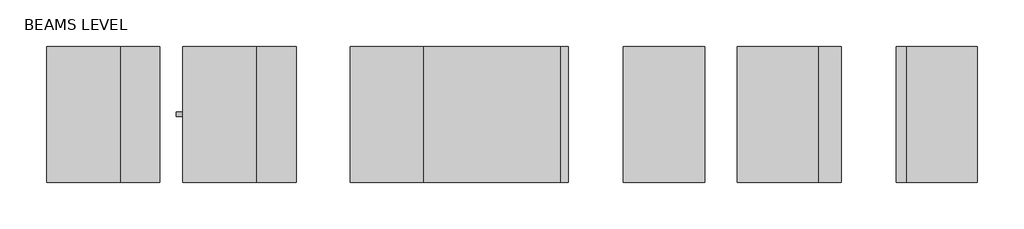
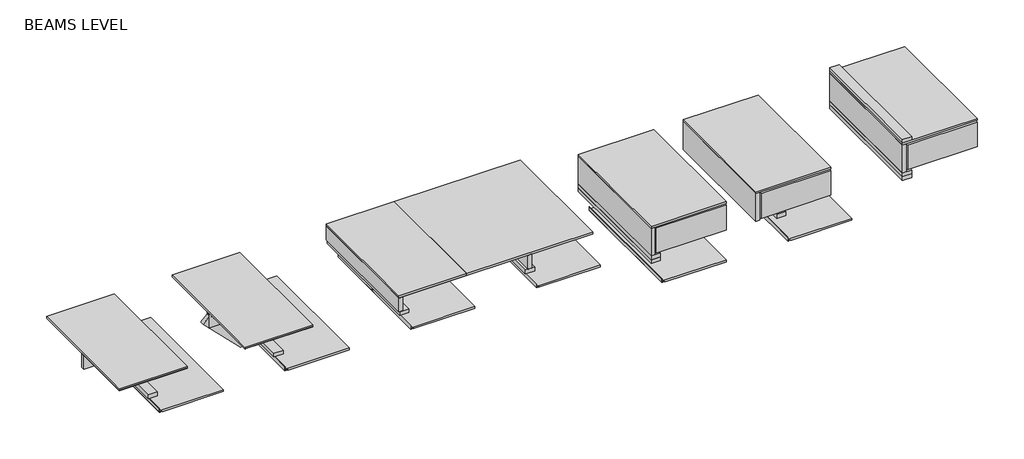
# One storey: 59 proxies.
"""IFC4 building model written with IfcOpenShell, lengths in millimetres."""

import ifcopenshell
import ifcopenshell.guid

model = None  # the IFC model being written
_history = None  # IfcOwnerHistory: only IFC2X3 demands one
_inside = {}  # id of a spatial element -> (the spatial element, [elements in it])
_under = {}  # id of a project, library or spatial element -> (it, [spatial elements below it])
_declared = {}  # id of a project -> (the project, [libraries it declares])
_typed = {}  # id of a type object -> (the type object, [elements of that type])
_made_of = {}  # id of a material, layer set ... -> (it, [elements and type objects made of it])


def new_model(schema):
    """Start an empty IFC model of exactly this schema.

    Asked for "IFC4X3", IfcOpenShell would pick the latest addendum, in which some entities
    have other attributes; the version numbers below select the first issue.
    IFC2X3 requires an IfcOwnerHistory on every rooted entity: one is made here for all.
    """
    global model, _history
    if schema == "IFC4X3":
        model = ifcopenshell.file(schema_version=(4, 3, 0, 0))
    else:
        model = ifcopenshell.file(schema=schema)
    _inside.clear()
    _under.clear()
    _declared.clear()
    _typed.clear()
    _made_of.clear()
    _history = None
    if model.schema == "IFC2X3":
        org = make("IfcOrganization", Name="unknown")
        user = make(
            "IfcPersonAndOrganization",
            ThePerson=make("IfcPerson", FamilyName="unknown"),
            TheOrganization=org,
        )
        app = make(
            "IfcApplication",
            ApplicationDeveloper=org,
            Version="unknown",
            ApplicationFullName="unknown",
            ApplicationIdentifier="unknown",
        )
        _history = make(
            "IfcOwnerHistory",
            OwningUser=user,
            OwningApplication=app,
            ChangeAction="ADDED",
            CreationDate=0,
        )
    return model


def make(cls, **values):
    """One entity of the class cls with the attributes given. An attribute that is None is left unset."""
    return model.create_entity(
        cls, **{name: value for name, value in values.items() if value is not None}
    )


def rooted(cls, **values):
    """An entity with a GlobalId (a new one), such as an element, a storey or a relation."""
    return make(cls, GlobalId=ifcopenshell.guid.new(), OwnerHistory=_history, **values)


def si_unit(unit_type, name, prefix=None):
    """IfcSIUnit, for example si_unit("LENGTHUNIT", "METRE", prefix="MILLI")."""
    return make("IfcSIUnit", UnitType=unit_type, Prefix=prefix, Name=name)


def assignment(units):
    """IfcUnitAssignment: the units of a project."""
    return None if units is None else make("IfcUnitAssignment", Units=units)


def point(xyz):
    """IfcCartesianPoint."""
    return None if xyz is None else make("IfcCartesianPoint", Coordinates=xyz)


def direction(xyz):
    """IfcDirection."""
    return None if xyz is None else make("IfcDirection", DirectionRatios=xyz)


def frame(location, z_axis=None, x_axis=None):
    """IfcAxis2Placement3D, a coordinate frame: its origin and axes. An axis left out is left unset."""
    return make(
        "IfcAxis2Placement3D",
        Location=point(location),
        Axis=direction(z_axis),
        RefDirection=direction(x_axis),
    )


def origin():
    """The frame at (0, 0, 0) with its axes left unset."""
    return frame((0.0, 0.0, 0.0))


def place(relative_to, where):
    """IfcLocalPlacement: puts the frame where relative to a parent placement (None: the world)."""
    return make(
        "IfcLocalPlacement", PlacementRelTo=relative_to, RelativePlacement=where
    )


def context(
    kind, dimensions, precision=None, world=None, true_north=None, identifier=None
):
    """IfcGeometricRepresentationContext, for example the 3D "Model" context."""
    return make(
        "IfcGeometricRepresentationContext",
        ContextIdentifier=identifier,
        ContextType=kind,
        CoordinateSpaceDimension=dimensions,
        Precision=precision,
        WorldCoordinateSystem=world,
        TrueNorth=true_north,
    )


def project(units=None, contexts=None):
    """IfcProject with its units and contexts."""
    return rooted(
        "IfcProject",
        Name="project",
        RepresentationContexts=contexts,
        UnitsInContext=assignment(units),
    )


def spatial(cls, under=None, at=None, **own):
    """A site, building, storey or space (cls), placed at a placement, below another one or the project."""
    s = rooted(cls, ObjectPlacement=at, **own)
    if under is not None:
        _under.setdefault(under.id(), (under, []))[1].append(s)
    return s


def polyline(points):
    """IfcPolyline through the points."""
    return make("IfcPolyline", Points=[point(p) for p in points])


def outline(outer, holes=None, kind="AREA"):
    """IfcArbitraryClosedProfileDef: a profile drawn as a closed curve; with holes, ...WithVoids."""
    if holes is None:
        return make("IfcArbitraryClosedProfileDef", ProfileType=kind, OuterCurve=outer)
    return make(
        "IfcArbitraryProfileDefWithVoids",
        ProfileType=kind,
        OuterCurve=outer,
        InnerCurves=holes,
    )


def extrude(swept, where, along, depth):
    """IfcExtrudedAreaSolid: the profile swept, set in the frame where, extruded along a direction by depth."""
    return make(
        "IfcExtrudedAreaSolid",
        SweptArea=swept,
        Position=where,
        ExtrudedDirection=direction(along),
        Depth=depth,
    )


def shape(context_of_items, identifier, shape_type, items):
    """IfcShapeRepresentation: the items that make up one representation, for example the "Body"."""
    return make(
        "IfcShapeRepresentation",
        ContextOfItems=context_of_items,
        RepresentationIdentifier=identifier,
        RepresentationType=shape_type,
        Items=items,
    )


def source(mapping_origin, context_of_items, identifier, shape_type, items):
    """IfcRepresentationMap: a shape defined once, which mapped items show again and again."""
    return make(
        "IfcRepresentationMap",
        MappingOrigin=mapping_origin,
        MappedRepresentation=shape(context_of_items, identifier, shape_type, items),
    )


def transform(
    local_origin,
    x_axis=None,
    y_axis=None,
    z_axis=None,
    scale=None,
    scale2=None,
    scale3=None,
    uniform=True,
):
    """IfcCartesianTransformationOperator3D, or its non-uniform kind. x_axis, y_axis, z_axis: its Axis1, 2, 3."""
    if uniform:
        return make(
            "IfcCartesianTransformationOperator3D",
            Axis1=direction(x_axis),
            Axis2=direction(y_axis),
            LocalOrigin=point(local_origin),
            Scale=scale,
            Axis3=direction(z_axis),
        )
    return make(
        "IfcCartesianTransformationOperator3DnonUniform",
        Axis1=direction(x_axis),
        Axis2=direction(y_axis),
        LocalOrigin=point(local_origin),
        Scale=scale,
        Axis3=direction(z_axis),
        Scale2=scale2,
        Scale3=scale3,
    )


def mapped(mapping_source, mapping_target):
    """IfcMappedItem: shows the shape of a source again, moved by a transform."""
    return make(
        "IfcMappedItem", MappingSource=mapping_source, MappingTarget=mapping_target
    )


def made_of(thing, what):
    """Note that an element or type object is made of a material, layer set ...; save() writes the relation."""
    if what is not None:
        _made_of.setdefault(what.id(), (what, []))[1].append(thing)
    return thing


def element(
    cls,
    number,
    at=None,
    inside=None,
    cuts=None,
    type_object=None,
    material=None,
    context=None,
    identifier="Body",
    shape_type=None,
    held_by="IfcProductDefinitionShape",
    body=None,
    shapes=None,
    **own,
):
    """One element of the class cls, such as IfcWall. Its Tag is "e" and its number.

    at: its placement. inside: the storey or other place that contains it. cuts: it is an
    opening in that element (IfcRelVoidsElement). A single representation is given by context,
    identifier, shape_type and body (its items); several are given by shapes. held_by: the class
    of the entity that holds the representations. save() writes the other relations.
    """
    e = rooted(cls, Tag="e%d" % number, ObjectPlacement=at, **own)
    if body is not None:
        shapes = [shape(context, identifier, shape_type, body)]
    if shapes is not None:
        e.Representation = make(held_by, Representations=shapes)
    if inside is not None:
        _inside.setdefault(inside.id(), (inside, []))[1].append(e)
    if cuts is not None:
        rooted(
            "IfcRelVoidsElement", RelatingBuildingElement=cuts, RelatedOpeningElement=e
        )
    if type_object is not None:
        _typed.setdefault(type_object.id(), (type_object, []))[1].append(e)
    return made_of(e, material)


def aggregate(whole, parts):
    """IfcRelAggregates: a whole, such as a stair, and the parts it consists of."""
    return rooted("IfcRelAggregates", RelatingObject=whole, RelatedObjects=parts)


def save(model, path):
    """Write the relations noted so far, then the file.

    IfcRelAggregates (storeys below a building ...), IfcRelContainedInSpatialStructure (elements
    in a storey), IfcRelDefinesByType, IfcRelAssociatesMaterial and IfcRelDeclares: one each for
    every whole, place, type object, material and project.
    """
    for whole, parts in _under.values():
        aggregate(whole, parts)
    for where, things in _inside.values():
        rooted(
            "IfcRelContainedInSpatialStructure",
            RelatedElements=things,
            RelatingStructure=where,
        )
    for kind, things in _typed.values():
        rooted("IfcRelDefinesByType", RelatedObjects=things, RelatingType=kind)
    for what, things in _made_of.values():
        rooted("IfcRelAssociatesMaterial", RelatedObjects=things, RelatingMaterial=what)
    for by, libraries in _declared.values():
        rooted("IfcRelDeclares", RelatingContext=by, RelatedDefinitions=libraries)
    model.write(path)


def generic_models_10_generic_models_1_ea081297(model_context):
    return source(origin(), model_context, "Body", "SweptSolid", [
        extrude(outline(polyline([(49758.6, 0.0), (49720.5, 0.0), (49720.5, 1219.2), (49758.6, 1219.2), (49758.6, 0.0)])), frame((0.0, 0.0, 5507.83125), z_axis=(0.0, 0.0, 1.0), x_axis=(1.0, 0.0, 0.0)), (0.0, 0.0, 1.0), 139.7),
    ])


def generic_models_109_generic_models_1_8619d77b(model_context):
    return source(origin(), model_context, "Body", "SweptSolid", [
        extrude(outline(polyline([(51003.2, 0.0), (50914.3, 0.0), (50914.3, 1219.2), (51003.2, 1219.2), (51003.2, 0.0)])), frame((0.0, 0.0, 5184.378125), z_axis=(0.0, 0.0, 1.0), x_axis=(1.0, 0.0, 0.0)), (0.0, 0.0, 1.0), 38.1),
    ])


def generic_models_110_generic_models_1_6bdce9b6(model_context):
    return source(origin(), model_context, "Body", "SweptSolid", [
        extrude(outline(polyline([(51642.1451407, 1219.2), (51642.1451407, 0.0), (50914.3, 0.0), (50914.3, 1219.2), (51642.1451407, 1219.2)])), frame((0.0, 0.0, 5508.228125), z_axis=(0.0, 0.0, 1.0), x_axis=(1.0, 0.0, 0.0)), (0.0, 0.0, 1.0), 19.05),
    ])


def generic_models_112_generic_models_65_d168d7b0(model_context):
    return source(origin(), model_context, "Body", "SweptSolid", [
        extrude(outline(polyline([(50952.4, 592.1375), (50952.4, 630.2375), (51642.1451407, 630.2375), (51642.1451407, 592.1375), (50952.4, 592.1375)])), frame((0.0, 0.0, 5222.478125), z_axis=(0.0, 0.0, 1.0), x_axis=(1.0, 0.0, 0.0)), (0.0, 0.0, 1.0), 285.75),
    ])


def generic_models_113_generic_models_1_101608ab(model_context):
    return source(origin(), model_context, "Body", "SweptSolid", [
        extrude(outline(polyline([(52171.6, 0.0), (52133.5, 0.0), (52133.5, 1219.2), (52171.6, 1219.2), (52171.6, 0.0)])), frame((0.0, 0.0, 5222.478125), z_axis=(0.0, 0.0, 1.0), x_axis=(1.0, 0.0, 0.0)), (0.0, 0.0, 1.0), 285.75),
    ])


def generic_models_114_generic_models_1_a6fb1c2c(model_context):
    return source(origin(), model_context, "Body", "SweptSolid", [
        extrude(outline(polyline([(51642.1451407, 1219.2), (51642.1451407, 0.0), (50965.9242022, 0.0), (50965.9242022, 1219.2), (51642.1451407, 1219.2)])), frame((0.0, 0.0, 5237.6235034), z_axis=(0.0, 0.0, 1.0), x_axis=(1.0, 0.0, 0.0)), (0.0, 0.0, 1.0), 254.0),
    ])


def generic_models_12_generic_models_46_b8a9a4e8(model_context):
    return source(origin(), model_context, "Body", "SweptSolid", [
        extrude(outline(polyline([(49757.8505137, 0.0), (49721.1284797, 0.0), (49721.1284797, 1219.2), (49757.8505137, 1219.2), (49757.8505137, 0.0)])), frame((0.0, 0.0, 5505.7509163), z_axis=(0.0, 0.0, 1.0), x_axis=(1.0, 0.0, 0.0)), (0.0, 0.0, 1.0), 1.5875),
    ])


def generic_models_13_generic_models_65_9e643fb9(model_context):
    return source(origin(), model_context, "Body", "SweptSolid", [
        extrude(outline(polyline([(49128.3625, 592.1375), (49128.3625, 630.2375), (50347.5625, 630.2375), (50347.5625, 592.1375), (49128.3625, 592.1375)])), frame((0.0, 0.0, 5507.83125), z_axis=(0.0, 0.0, 1.0), x_axis=(1.0, 0.0, 0.0)), (0.0, 0.0, 1.0), 139.7),
    ])


def generic_models_14_generic_models_1_e8c90d4c(model_context):
    return source(origin(), model_context, "Body", "SweptSolid", [
        extrude(outline(polyline([(2277.1204978, 49799.875), (2239.0204978, 49799.875), (2239.0204978, 49825.275), (2240.6079978, 49825.275), (2240.6079978, 49801.4625), (2277.1204978, 49801.4625), (2277.1204978, 49799.875)])), frame((0.0, 0.0, 0.0), z_axis=(0.0, 1.0, 0.0), x_axis=(0.0, 0.0, 1.0)), (0.0, 0.0, 1.0), 1219.2),
    ])


def generic_models_22_generic_models_1_e5767157(model_context):
    return source(origin(), model_context, "Body", "SweptSolid", [
        extrude(outline(polyline([(2409.6091, 49800.66875), (2409.6091, 49799.875), (2407.0592364, 49799.875), (2405.4618473, 49749.075), (2404.6631527, 49749.075), (2403.0657636, 49799.875), (2400.5159, 49799.875), (2400.5159, 49800.66875), (2409.6091, 49800.66875)])), frame((0.0, 565.15, 0.0), z_axis=(0.0, 1.0, 0.0), x_axis=(0.0, 0.0, 1.0)), (0.0, 0.0, 1.0), 12.7),
    ])


def generic_models_226_generic_models_1_7dc37832(model_context):
    return source(origin(), model_context, "Body", "SweptSolid", [
        extrude(outline(polyline([(5263.35625, 49733.4159), (5263.35625, 49742.5091), (5264.15, 49742.5091), (5264.15, 49739.9592364), (5314.95, 49738.3618473), (5314.95, 49737.5631527), (5264.15, 49735.9657636), (5264.15, 49733.4159), (5263.35625, 49733.4159)])), frame((0.0, 565.15, 0.0), z_axis=(0.0, 1.0, 0.0), x_axis=(0.0, 0.0, 1.0)), (0.0, 0.0, 1.0), 12.7),
    ])


def generic_models_202_generic_models_1_0ad20a8b(model_context):
    return source(origin(), model_context, "Body", "SweptSolid", [
        extrude(outline(polyline([(2253.330428, 49813.3451407), (2242.217928, 49813.3451407), (2242.217928, 49826.0451407), (2234.280428, 49828.9341545), (2234.280428, 50422.9451407), (2253.330428, 50422.9451407), (2253.330428, 49813.3451407)])), frame((0.0, 0.0, 0.0), z_axis=(0.0, 1.0, 0.0), x_axis=(0.0, 0.0, 1.0)), (0.0, 0.0, 1.0), 1219.2),
    ])


def generic_models_233_generic_models_1_ae5bae41(model_context):
    return source(origin(), model_context, "Body", "SweptSolid", [
        extrude(outline(polyline([(48564.8, 0.0), (48475.9, 0.0), (48475.9, 1219.2), (48564.8, 1219.2), (48564.8, 0.0)])), frame((0.0, 0.0, 5467.35), z_axis=(0.0, 0.0, 1.0), x_axis=(1.0, 0.0, 0.0)), (0.0, 0.0, 1.0), 38.1),
    ])


def generic_models_236_generic_models_1_f8917e71(model_context):
    return source(origin(), model_context, "Body", "SweptSolid", [
        extrude(outline(polyline([(48507.65, 0.0), (48469.55, 0.0), (48469.55, 1219.2), (48507.65, 1219.2), (48507.65, 0.0)])), frame((0.0, 0.0, 5507.83125), z_axis=(0.0, 0.0, 1.0), x_axis=(1.0, 0.0, 0.0)), (0.0, 0.0, 1.0), 139.7),
    ])


def generic_models_237_generic_models_65_1df05f16(model_context):
    return source(origin(), model_context, "Body", "SweptSolid", [
        extrude(outline(polyline([(48469.55, 592.1375), (48469.55, 630.2375), (49128.3625, 630.2375), (49128.3625, 592.1375), (48469.55, 592.1375)])), frame((0.0, 0.0, 5507.83125), z_axis=(0.0, 0.0, 1.0), x_axis=(1.0, 0.0, 0.0)), (0.0, 0.0, 1.0), 139.7),
    ])


def generic_models_239_generic_models_46_95e6735a(model_context):
    return source(origin(), model_context, "Body", "SweptSolid", [
        extrude(outline(polyline([(50347.5625, 0.0), (49691.4320511, 0.0), (49691.4320511, 1219.2), (50347.5625, 1219.2), (50347.5625, 0.0)])), frame((0.0, 0.0, 5505.7509163), z_axis=(0.0, 0.0, 1.0), x_axis=(1.0, 0.0, 0.0)), (0.0, 0.0, 1.0), 1.5875),
    ])


def generic_models_240_generic_models_1_611786cf(model_context):
    return source(origin(), model_context, "Body", "SweptSolid", [
        extrude(outline(polyline([(49128.3625, 1219.2), (49128.3625, 0.0), (48469.55, 0.0), (48469.55, 1219.2), (49128.3625, 1219.2)])), frame((0.0, 0.0, 5649.9125), z_axis=(0.0, 0.0, 1.0), x_axis=(1.0, 0.0, 0.0)), (0.0, 0.0, 1.0), 19.05),
    ])


def generic_models_267_generic_models_65_11354230(model_context):
    return source(origin(), model_context, "Body", "SweptSolid", [
        extrude(outline(polyline([(0.0, -38.1), (0.0, 0.0), (514.35, 0.0), (514.35, -38.1), (0.0, -38.1)])), frame((47276.4596037, 592.1375, 5202.484661), z_axis=(0.7071067811865633, 0.0, 0.7071067811865317), x_axis=(-0.7071067811865317, 0.0, 0.7071067811865633)), (0.0, 0.0, 1.0), 88.9),
    ])


def generic_models_29_generic_models_1_59087225(model_context):
    return source(origin(), model_context, "Body", "SweptSolid", [
        extrude(outline(polyline([(50347.5625, 1219.2), (50347.5625, 0.0), (49128.3625, 0.0), (49128.3625, 1219.2), (50347.5625, 1219.2)])), frame((0.0, 0.0, 5647.53125), z_axis=(0.0, 0.0, 1.0), x_axis=(1.0, 0.0, 0.0)), (0.0, 0.0, 1.0), 19.05),
    ])


def generic_models_37_generic_models_1_916dd7c6(model_context):
    return source(origin(), model_context, "Body", "SweptSolid", [
        extrude(outline(polyline([(2409.6091, 49675.25625), (2400.5159, 49675.25625), (2400.5159, 49676.05), (2403.0657636, 49676.05), (2404.6631527, 49726.85), (2405.4618473, 49726.85), (2407.0592364, 49676.05), (2409.6091, 49676.05), (2409.6091, 49675.25625)])), frame((0.0, 565.15, 0.0), z_axis=(0.0, 1.0, 0.0), x_axis=(0.0, 0.0, 1.0)), (0.0, 0.0, 1.0), 12.7),
    ])


def generic_models_103_generic_models_1_250a6a11(model_context):
    return source(origin(), model_context, "Body", "SweptSolid", [
        extrude(outline(polyline([(49784.0, 0.0), (49695.1, 0.0), (49695.1, 1219.2), (49784.0, 1219.2), (49784.0, 0.0)])), frame((0.0, 0.0, 5264.15), z_axis=(0.0, 0.0, 1.0), x_axis=(1.0, 0.0, 0.0)), (0.0, 0.0, 1.0), 38.1),
    ])


def generic_models_71_generic_models_1_508a995f(model_context):
    return source(origin(), model_context, "Body", "SweptSolid", [
        extrude(outline(polyline([(50952.4, 0.0), (50914.3, 0.0), (50914.3, 1219.2), (50952.4, 1219.2), (50952.4, 0.0)])), frame((0.0, 0.0, 5222.478125), z_axis=(0.0, 0.0, 1.0), x_axis=(1.0, 0.0, 0.0)), (0.0, 0.0, 1.0), 285.75),
    ])


def generic_models_87_generic_models_1_55a64953(model_context):
    return source(origin(), model_context, "Body", "SweptSolid", [
        extrude(outline(polyline([(51968.4, 0.0), (51930.3, 0.0), (51930.3, 1219.2), (51968.4, 1219.2), (51968.4, 0.0)])), frame((0.0, 0.0, 5222.478125), z_axis=(0.0, 0.0, 1.0), x_axis=(1.0, 0.0, 0.0)), (0.0, 0.0, 1.0), 285.75),
    ])


model = new_model("IFC4")

# Units and contexts
model_context = context("Model", 3, world=origin())
ifc_project = project(units=[si_unit("LENGTHUNIT", "METRE", prefix="MILLI")], contexts=[model_context])

# Site, building, storey
site = spatial("IfcSite", under=ifc_project)
building = spatial("IfcBuilding", under=site)
storey = spatial("IfcBuildingStorey", under=building, Name="BEAMS LEVEL", Elevation=4876.8)

# Proxies
placement = place(None, origin())
generic_models_10_generic_models_1_shape = generic_models_10_generic_models_1_ea081297(model_context)
element("IfcBuildingElementProxy", 1, Name="Generic Models 10 : Generic Models 1", ObjectType="Generic Models 10 : Generic Models 1", at=placement, inside=storey, context=model_context, shape_type="MappedRepresentation", body=[
    mapped(generic_models_10_generic_models_1_shape, transform((0.0, 0.0, 0.0), x_axis=(1.0, 0.0, 0.0), y_axis=(0.0, 1.0, 0.0), z_axis=(0.0, 0.0, 1.0))),
])
generic_models_109_generic_models_1_shape = generic_models_109_generic_models_1_8619d77b(model_context)
element("IfcBuildingElementProxy", 2, Name="Generic Models 109 : Generic Models 1", ObjectType="Generic Models 109 : Generic Models 1", at=placement, inside=storey, context=model_context, shape_type="MappedRepresentation", body=[
    mapped(generic_models_109_generic_models_1_shape, transform((2438.4, 0.0, 0.0), x_axis=(1.0, 0.0, 0.0), y_axis=(0.0, 1.0, 0.0), z_axis=(0.0, 0.0, 1.0))),
])
generic_models_110_generic_models_1_shape = generic_models_110_generic_models_1_6bdce9b6(model_context)
element("IfcBuildingElementProxy", 3, Name="Generic Models 110 : Generic Models 1", ObjectType="Generic Models 110 : Generic Models 1", at=placement, inside=storey, context=model_context, shape_type="MappedRepresentation", body=[
    mapped(generic_models_110_generic_models_1_shape, transform((2438.4, 0.0, 0.0), x_axis=(1.0, 0.0, 0.0), y_axis=(0.0, 1.0, 0.0), z_axis=(0.0, 0.0, 1.0))),
])
element("IfcBuildingElementProxy", 4, Name="Generic Models 111 : Generic Models 1", ObjectType="Generic Models 111 : Generic Models 1", at=placement, inside=storey, context=model_context, shape_type="MappedRepresentation", body=[
    mapped(generic_models_109_generic_models_1_shape, transform((2438.4, 0.0, -38.1), x_axis=(1.0, 0.0, 0.0), y_axis=(0.0, 1.0, 0.0), z_axis=(0.0, 0.0, 1.0))),
])
generic_models_112_generic_models_65_shape = generic_models_112_generic_models_65_d168d7b0(model_context)
element("IfcBuildingElementProxy", 5, Name="Generic Models 112 : Generic Models 65", ObjectType="Generic Models 112 : Generic Models 65", at=placement, inside=storey, context=model_context, shape_type="MappedRepresentation", body=[
    mapped(generic_models_112_generic_models_65_shape, transform((2438.4, 0.0, 0.0), x_axis=(1.0, 0.0, 0.0), y_axis=(0.0, 1.0, 0.0), z_axis=(0.0, 0.0, 1.0))),
])
generic_models_113_generic_models_1_shape = generic_models_113_generic_models_1_101608ab(model_context)
element("IfcBuildingElementProxy", 6, Name="Generic Models 113 : Generic Models 1", ObjectType="Generic Models 113 : Generic Models 1", at=placement, inside=storey, context=model_context, shape_type="MappedRepresentation", body=[
    mapped(generic_models_113_generic_models_1_shape, transform((1219.2, 0.0, 0.0), x_axis=(1.0, 0.0, 0.0), y_axis=(0.0, 1.0, 0.0), z_axis=(0.0, 0.0, 1.0))),
])
generic_models_114_generic_models_1_shape = generic_models_114_generic_models_1_a6fb1c2c(model_context)
element("IfcBuildingElementProxy", 7, Name="Generic Models 114 : Generic Models 1", ObjectType="Generic Models 114 : Generic Models 1", at=placement, inside=storey, context=model_context, shape_type="MappedRepresentation", body=[
    mapped(generic_models_114_generic_models_1_shape, transform((2438.4, 0.0, 0.0), x_axis=(1.0, 0.0, 0.0), y_axis=(0.0, 1.0, 0.0), z_axis=(0.0, 0.0, 1.0))),
])
element("IfcBuildingElementProxy", 8, Name="Generic Models 115 : Generic Models 1", ObjectType="Generic Models 115 : Generic Models 1", at=placement, inside=storey, context=model_context, shape_type="MappedRepresentation", body=[
    mapped(generic_models_109_generic_models_1_shape, transform((2438.4, 0.0, 342.9), x_axis=(1.0, 0.0, 0.0), y_axis=(0.0, 1.0, 0.0), z_axis=(0.0, 0.0, 1.0))),
])
generic_models_12_generic_models_46_shape = generic_models_12_generic_models_46_b8a9a4e8(model_context)
element("IfcBuildingElementProxy", 9, Name="Generic Models 12 : Generic Models 46", ObjectType="Generic Models 12 : Generic Models 46", at=placement, inside=storey, context=model_context, shape_type="MappedRepresentation", body=[
    mapped(generic_models_12_generic_models_46_shape, transform((0.0, 0.0, 0.0), x_axis=(1.0, 0.0, 0.0), y_axis=(0.0, 1.0, 0.0), z_axis=(0.0, 0.0, 1.0))),
])
generic_models_13_generic_models_65_shape = generic_models_13_generic_models_65_9e643fb9(model_context)
element("IfcBuildingElementProxy", 10, Name="Generic Models 13 : Generic Models 65", ObjectType="Generic Models 13 : Generic Models 65", at=placement, inside=storey, context=model_context, shape_type="MappedRepresentation", body=[
    mapped(generic_models_13_generic_models_65_shape, transform((0.0, 0.0, 0.0), x_axis=(1.0, 0.0, 0.0), y_axis=(0.0, 1.0, 0.0), z_axis=(0.0, 0.0, 1.0))),
])
generic_models_14_generic_models_1_shape = generic_models_14_generic_models_1_e8c90d4c(model_context)
element("IfcBuildingElementProxy", 11, Name="Generic Models 14 : Generic Models 1", ObjectType="Generic Models 14 : Generic Models 1", at=placement, inside=storey, context=model_context, shape_type="MappedRepresentation", body=[
    mapped(generic_models_14_generic_models_1_shape, transform((0.0, 0.0, 3050.778125), x_axis=(1.0, 0.0, 0.0), y_axis=(0.0, 1.0, 0.0), z_axis=(0.0, 0.0, 1.0))),
])
generic_models_22_generic_models_1_shape = generic_models_22_generic_models_1_e5767157(model_context)
element("IfcBuildingElementProxy", 12, Name="Generic Models 22 : Generic Models 1", ObjectType="Generic Models 22 : Generic Models 1", at=placement, inside=storey, context=model_context, shape_type="MappedRepresentation", body=[
    mapped(generic_models_22_generic_models_1_shape, transform((0.0, 0.0, 3081.3375), x_axis=(1.0, 0.0, 0.0), y_axis=(0.0, 1.0, 0.0), z_axis=(0.0, 0.0, 1.0))),
])
element("IfcBuildingElementProxy", 13, Name="Generic Models 224 : Generic Models 1", ObjectType="Generic Models 224 : Generic Models 1", at=placement, inside=storey, context=model_context, shape_type="MappedRepresentation", body=[
    mapped(generic_models_14_generic_models_1_shape, transform((-1217.6125, 0.0, 3050.778125), x_axis=(1.0, 0.0, 0.0), y_axis=(0.0, 1.0, 0.0), z_axis=(0.0, 0.0, 1.0))),
])
element("IfcBuildingElementProxy", 14, Name="Generic Models 225 : Generic Models 1", ObjectType="Generic Models 225 : Generic Models 1", at=placement, inside=storey, context=model_context, shape_type="MappedRepresentation", body=[
    mapped(generic_models_22_generic_models_1_shape, transform((-1219.2, 0.0, 2960.6875), x_axis=(1.0, 0.0, 0.0), y_axis=(0.0, 1.0, 0.0), z_axis=(0.0, 0.0, 1.0))),
])
generic_models_226_generic_models_1_shape = generic_models_226_generic_models_1_7dc37832(model_context)
element("IfcBuildingElementProxy", 15, Name="Generic Models 226 : Generic Models 1", ObjectType="Generic Models 226 : Generic Models 1", at=placement, inside=storey, context=model_context, shape_type="MappedRepresentation", body=[
    mapped(generic_models_226_generic_models_1_shape, transform((-1219.2, 0.0, 203.2), x_axis=(1.0, 0.0, 0.0), y_axis=(0.0, 1.0, 0.0), z_axis=(0.0, 0.0, 1.0))),
])
generic_models_202_generic_models_1_shape = generic_models_202_generic_models_1_0ad20a8b(model_context)
element("IfcBuildingElementProxy", 16, Name="Generic Models 231 : Generic Models 1", ObjectType="Generic Models 231 : Generic Models 1", at=placement, inside=storey, context=model_context, shape_type="MappedRepresentation", body=[
    mapped(generic_models_202_generic_models_1_shape, transform((-1217.6125, 0.0, 3050.778125), x_axis=(1.0, 0.0, 0.0), y_axis=(0.0, 1.0, 0.0), z_axis=(0.0, 0.0, 1.0))),
])
generic_models_233_generic_models_1_shape = generic_models_233_generic_models_1_ae5bae41(model_context)
element("IfcBuildingElementProxy", 17, Name="Generic Models 233 : Generic Models 1", ObjectType="Generic Models 233 : Generic Models 1", at=placement, inside=storey, context=model_context, shape_type="MappedRepresentation", body=[
    mapped(generic_models_233_generic_models_1_shape, transform((0.0, 0.0, 0.0), x_axis=(1.0, 0.0, 0.0), y_axis=(0.0, 1.0, 0.0), z_axis=(0.0, 0.0, 1.0))),
])
generic_models_236_generic_models_1_shape = generic_models_236_generic_models_1_f8917e71(model_context)
element("IfcBuildingElementProxy", 18, Name="Generic Models 236 : Generic Models 1", ObjectType="Generic Models 236 : Generic Models 1", at=placement, inside=storey, context=model_context, shape_type="MappedRepresentation", body=[
    mapped(generic_models_236_generic_models_1_shape, transform((0.0, 0.0, 0.0), x_axis=(1.0, 0.0, 0.0), y_axis=(0.0, 1.0, 0.0), z_axis=(0.0, 0.0, 1.0))),
])
generic_models_237_generic_models_65_shape = generic_models_237_generic_models_65_1df05f16(model_context)
element("IfcBuildingElementProxy", 19, Name="Generic Models 237 : Generic Models 65", ObjectType="Generic Models 237 : Generic Models 65", at=placement, inside=storey, context=model_context, shape_type="MappedRepresentation", body=[
    mapped(generic_models_237_generic_models_65_shape, transform((0.0, 0.0, 0.0), x_axis=(1.0, 0.0, 0.0), y_axis=(0.0, 1.0, 0.0), z_axis=(0.0, 0.0, 1.0))),
])
element("IfcBuildingElementProxy", 20, Name="Generic Models 238 : Generic Models 1", ObjectType="Generic Models 238 : Generic Models 1", at=placement, inside=storey, context=model_context, shape_type="MappedRepresentation", body=[
    mapped(generic_models_14_generic_models_1_shape, transform((-3656.0125, 0.0, 3050.778125), x_axis=(1.0, 0.0, 0.0), y_axis=(0.0, 1.0, 0.0), z_axis=(0.0, 0.0, 1.0))),
])
generic_models_239_generic_models_46_shape = generic_models_239_generic_models_46_95e6735a(model_context)
element("IfcBuildingElementProxy", 21, Name="Generic Models 239 : Generic Models 46", ObjectType="Generic Models 239 : Generic Models 46", at=placement, inside=storey, context=model_context, shape_type="MappedRepresentation", body=[
    mapped(generic_models_239_generic_models_46_shape, transform((-1219.2, 0.0, 142.08125), x_axis=(1.0, 0.0, 0.0), y_axis=(0.0, 1.0, 0.0), z_axis=(0.0, 0.0, 1.0))),
])
generic_models_240_generic_models_1_shape = generic_models_240_generic_models_1_611786cf(model_context)
element("IfcBuildingElementProxy", 22, Name="Generic Models 240 : Generic Models 1", ObjectType="Generic Models 240 : Generic Models 1", at=placement, inside=storey, context=model_context, shape_type="MappedRepresentation", body=[
    mapped(generic_models_240_generic_models_1_shape, transform((0.0, 0.0, 0.0), x_axis=(1.0, 0.0, 0.0), y_axis=(0.0, 1.0, 0.0), z_axis=(0.0, 0.0, 1.0))),
])
element("IfcBuildingElementProxy", 23, Name="Generic Models 242 : Generic Models 1", ObjectType="Generic Models 242 : Generic Models 1", at=placement, inside=storey, context=model_context, shape_type="MappedRepresentation", body=[
    mapped(generic_models_22_generic_models_1_shape, transform((-3657.6, 0.0, 2960.6875), x_axis=(1.0, 0.0, 0.0), y_axis=(0.0, 1.0, 0.0), z_axis=(0.0, 0.0, 1.0))),
])
element("IfcBuildingElementProxy", 24, Name="Generic Models 243 : Generic Models 1", ObjectType="Generic Models 243 : Generic Models 1", at=placement, inside=storey, context=model_context, shape_type="MappedRepresentation", body=[
    mapped(generic_models_226_generic_models_1_shape, transform((-3656.0125, 0.0, 203.2), x_axis=(1.0, 0.0, 0.0), y_axis=(0.0, 1.0, 0.0), z_axis=(0.0, 0.0, 1.0))),
])
element("IfcBuildingElementProxy", 25, Name="Generic Models 245 : Generic Models 1", ObjectType="Generic Models 245 : Generic Models 1", at=placement, inside=storey, context=model_context, shape_type="MappedRepresentation", body=[
    mapped(generic_models_202_generic_models_1_shape, transform((-3656.0125, 0.0, 3050.778125), x_axis=(1.0, 0.0, 0.0), y_axis=(0.0, 1.0, 0.0), z_axis=(0.0, 0.0, 1.0))),
])
element("IfcBuildingElementProxy", 26, Name="Generic Models 247 : Generic Models 1", ObjectType="Generic Models 247 : Generic Models 1", at=placement, inside=storey, context=model_context, shape_type="MappedRepresentation", body=[
    mapped(generic_models_233_generic_models_1_shape, transform((-2438.4, 0.0, 0.0), x_axis=(1.0, 0.0, 0.0), y_axis=(0.0, 1.0, 0.0), z_axis=(0.0, 0.0, 1.0))),
])
element("IfcBuildingElementProxy", 27, Name="Generic Models 25 : Generic Models 46", ObjectType="Generic Models 25 : Generic Models 46", at=placement, inside=storey, context=model_context, shape_type="MappedRepresentation", body=[
    mapped(generic_models_12_generic_models_46_shape, transform((0.0, 0.0, 142.08125), x_axis=(1.0, 0.0, 0.0), y_axis=(0.0, 1.0, 0.0), z_axis=(0.0, 0.0, 1.0))),
])
element("IfcBuildingElementProxy", 28, Name="Generic Models 250 : Generic Models 65", ObjectType="Generic Models 250 : Generic Models 65", at=placement, inside=storey, context=model_context, shape_type="MappedRepresentation", body=[
    mapped(generic_models_237_generic_models_65_shape, transform((-2714.8439208, 0.0, 0.0), x_axis=(1.0, 0.0, 0.0), y_axis=(0.0, 1.0, 0.0), z_axis=(0.0, 0.0, 1.0))),
])
element("IfcBuildingElementProxy", 29, Name="Generic Models 251 : Generic Models 46", ObjectType="Generic Models 251 : Generic Models 46", at=placement, inside=storey, context=model_context, shape_type="MappedRepresentation", body=[
    mapped(generic_models_239_generic_models_46_shape, transform((-3934.0439208, 0.0, 142.08125), x_axis=(1.0, 0.0, 0.0), y_axis=(0.0, 1.0, 0.0), z_axis=(0.0, 0.0, 1.0))),
])
element("IfcBuildingElementProxy", 30, Name="Generic Models 252 : Generic Models 1", ObjectType="Generic Models 252 : Generic Models 1", at=placement, inside=storey, context=model_context, shape_type="MappedRepresentation", body=[
    mapped(generic_models_240_generic_models_1_shape, transform((-2714.8439208, 0.0, 0.0), x_axis=(1.0, 0.0, 0.0), y_axis=(0.0, 1.0, 0.0), z_axis=(0.0, 0.0, 1.0))),
])
element("IfcBuildingElementProxy", 31, Name="Generic Models 255 : Generic Models 1", ObjectType="Generic Models 255 : Generic Models 1", at=placement, inside=storey, context=model_context, shape_type="MappedRepresentation", body=[
    mapped(generic_models_14_generic_models_1_shape, transform((-2436.8125, 0.0, 3050.778125), x_axis=(1.0, 0.0, 0.0), y_axis=(0.0, 1.0, 0.0), z_axis=(0.0, 0.0, 1.0))),
])
element("IfcBuildingElementProxy", 32, Name="Generic Models 256 : Generic Models 1", ObjectType="Generic Models 256 : Generic Models 1", at=placement, inside=storey, context=model_context, shape_type="MappedRepresentation", body=[
    mapped(generic_models_22_generic_models_1_shape, transform((-2438.4, 0.0, 2960.6875), x_axis=(1.0, 0.0, 0.0), y_axis=(0.0, 1.0, 0.0), z_axis=(0.0, 0.0, 1.0))),
])
element("IfcBuildingElementProxy", 33, Name="Generic Models 257 : Generic Models 1", ObjectType="Generic Models 257 : Generic Models 1", at=placement, inside=storey, context=model_context, shape_type="MappedRepresentation", body=[
    mapped(generic_models_226_generic_models_1_shape, transform((-2438.4, 0.0, 203.2), x_axis=(1.0, 0.0, 0.0), y_axis=(0.0, 1.0, 0.0), z_axis=(0.0, 0.0, 1.0))),
])
element("IfcBuildingElementProxy", 34, Name="Generic Models 259 : Generic Models 1", ObjectType="Generic Models 259 : Generic Models 1", at=placement, inside=storey, context=model_context, shape_type="MappedRepresentation", body=[
    mapped(generic_models_202_generic_models_1_shape, transform((-2436.8125, 0.0, 3050.778125), x_axis=(1.0, 0.0, 0.0), y_axis=(0.0, 1.0, 0.0), z_axis=(0.0, 0.0, 1.0))),
])
element("IfcBuildingElementProxy", 35, Name="Generic Models 261 : Generic Models 1", ObjectType="Generic Models 261 : Generic Models 1", at=placement, inside=storey, context=model_context, shape_type="MappedRepresentation", body=[
    mapped(generic_models_233_generic_models_1_shape, transform((-1219.2, 0.0, 0.0), x_axis=(1.0, 0.0, 0.0), y_axis=(0.0, 1.0, 0.0), z_axis=(0.0, 0.0, 1.0))),
])
element("IfcBuildingElementProxy", 36, Name="Generic Models 264 : Generic Models 65", ObjectType="Generic Models 264 : Generic Models 65", at=placement, inside=storey, context=model_context, shape_type="MappedRepresentation", body=[
    mapped(generic_models_237_generic_models_65_shape, transform((-1497.80625, 0.0, 0.0), x_axis=(1.0, 0.0, 0.0), y_axis=(0.0, 1.0, 0.0), z_axis=(0.0, 0.0, 1.0))),
])
element("IfcBuildingElementProxy", 37, Name="Generic Models 265 : Generic Models 46", ObjectType="Generic Models 265 : Generic Models 46", at=placement, inside=storey, context=model_context, shape_type="MappedRepresentation", body=[
    mapped(generic_models_239_generic_models_46_shape, transform((-2717.00625, 0.0, 142.08125), x_axis=(1.0, 0.0, 0.0), y_axis=(0.0, 1.0, 0.0), z_axis=(0.0, 0.0, 1.0))),
])
element("IfcBuildingElementProxy", 38, Name="Generic Models 266 : Generic Models 1", ObjectType="Generic Models 266 : Generic Models 1", at=placement, inside=storey, context=model_context, shape_type="MappedRepresentation", body=[
    mapped(generic_models_240_generic_models_1_shape, transform((-1497.80625, 0.0, 0.0), x_axis=(1.0, 0.0, 0.0), y_axis=(0.0, 1.0, 0.0), z_axis=(0.0, 0.0, 1.0))),
])
generic_models_267_generic_models_65_shape = generic_models_267_generic_models_65_11354230(model_context)
element("IfcBuildingElementProxy", 39, Name="Generic Models 267 : Generic Models 65", ObjectType="Generic Models 267 : Generic Models 65", at=placement, inside=storey, context=model_context, shape_type="MappedRepresentation", body=[
    mapped(generic_models_267_generic_models_65_shape, transform((0.0, 0.0, 0.0), x_axis=(1.0, 0.0, 0.0), y_axis=(0.0, 1.0, 0.0), z_axis=(0.0, 0.0, 1.0))),
])
generic_models_29_generic_models_1_shape = generic_models_29_generic_models_1_59087225(model_context)
element("IfcBuildingElementProxy", 40, Name="Generic Models 29 : Generic Models 1", ObjectType="Generic Models 29 : Generic Models 1", at=placement, inside=storey, context=model_context, shape_type="MappedRepresentation", body=[
    mapped(generic_models_29_generic_models_1_shape, transform((0.0, 0.0, 2.38125), x_axis=(1.0, 0.0, 0.0), y_axis=(0.0, 1.0, 0.0), z_axis=(0.0, 0.0, 1.0))),
])
element("IfcBuildingElementProxy", 41, Name="Generic Models 39 : Generic Models 1", ObjectType="Generic Models 39 : Generic Models 1", at=placement, inside=storey, context=model_context, shape_type="MappedRepresentation", body=[
    mapped(generic_models_226_generic_models_1_shape, transform((0.0, 0.0, 203.2), x_axis=(1.0, 0.0, 0.0), y_axis=(0.0, 1.0, 0.0), z_axis=(0.0, 0.0, 1.0))),
])
generic_models_37_generic_models_1_shape = generic_models_37_generic_models_1_916dd7c6(model_context)
element("IfcBuildingElementProxy", 42, Name="Generic Models 47 : Generic Models 1", ObjectType="Generic Models 47 : Generic Models 1", at=placement, inside=storey, context=model_context, shape_type="MappedRepresentation", body=[
    mapped(generic_models_37_generic_models_1_shape, transform((3.175, 0.0, 3081.3375), x_axis=(1.0, 0.0, 0.0), y_axis=(0.0, 1.0, 0.0), z_axis=(0.0, 0.0, 1.0))),
])
element("IfcBuildingElementProxy", 43, Name="Generic Models 49 : Generic Models 1", ObjectType="Generic Models 49 : Generic Models 1", at=placement, inside=storey, context=model_context, shape_type="MappedRepresentation", body=[
    mapped(generic_models_202_generic_models_1_shape, transform((0.0, 0.0, 3050.778125), x_axis=(1.0, 0.0, 0.0), y_axis=(0.0, 1.0, 0.0), z_axis=(0.0, 0.0, 1.0))),
])
element("IfcBuildingElementProxy", 44, Name="Generic Models 54 : Generic Models 1", ObjectType="Generic Models 54 : Generic Models 1", at=placement, inside=storey, context=model_context, shape_type="MappedRepresentation", body=[
    mapped(generic_models_14_generic_models_1_shape, transform((1219.2, 0.0, 2676.128125), x_axis=(1.0, 0.0, 0.0), y_axis=(0.0, 1.0, 0.0), z_axis=(0.0, 0.0, 1.0))),
])
element("IfcBuildingElementProxy", 45, Name="Generic Models 59 : Generic Models 65", ObjectType="Generic Models 59 : Generic Models 65", at=placement, inside=storey, context=model_context, shape_type="MappedRepresentation", body=[
    mapped(generic_models_112_generic_models_65_shape, transform((0.0, 0.0, 0.0), x_axis=(1.0, 0.0, 0.0), y_axis=(0.0, 1.0, 0.0), z_axis=(0.0, 0.0, 1.0))),
])
generic_models_103_generic_models_1_shape = generic_models_103_generic_models_1_250a6a11(model_context)
element("IfcBuildingElementProxy", 46, Name="Generic Models 6 : Generic Models 1", ObjectType="Generic Models 6 : Generic Models 1", at=placement, inside=storey, context=model_context, shape_type="MappedRepresentation", body=[
    mapped(generic_models_103_generic_models_1_shape, transform((0.0, 0.0, 203.2), x_axis=(1.0, 0.0, 0.0), y_axis=(0.0, 1.0, 0.0), z_axis=(0.0, 0.0, 1.0))),
])
element("IfcBuildingElementProxy", 47, Name="Generic Models 62 : Generic Models 1", ObjectType="Generic Models 62 : Generic Models 1", at=placement, inside=storey, context=model_context, shape_type="MappedRepresentation", body=[
    mapped(generic_models_202_generic_models_1_shape, transform((1219.2, 0.0, 2676.128125), x_axis=(1.0, 0.0, 0.0), y_axis=(0.0, 1.0, 0.0), z_axis=(0.0, 0.0, 1.0))),
])
element("IfcBuildingElementProxy", 48, Name="Generic Models 64 : Generic Models 1", ObjectType="Generic Models 64 : Generic Models 1", at=placement, inside=storey, context=model_context, shape_type="MappedRepresentation", body=[
    mapped(generic_models_109_generic_models_1_shape, transform((0.0, 0.0, 0.0), x_axis=(1.0, 0.0, 0.0), y_axis=(0.0, 1.0, 0.0), z_axis=(0.0, 0.0, 1.0))),
])
element("IfcBuildingElementProxy", 49, Name="Generic Models 66 : Generic Models 1", ObjectType="Generic Models 66 : Generic Models 1", at=placement, inside=storey, context=model_context, shape_type="MappedRepresentation", body=[
    mapped(generic_models_110_generic_models_1_shape, transform((0.0, 0.0, 0.0), x_axis=(1.0, 0.0, 0.0), y_axis=(0.0, 1.0, 0.0), z_axis=(0.0, 0.0, 1.0))),
])
element("IfcBuildingElementProxy", 50, Name="Generic Models 70 : Generic Models 1", ObjectType="Generic Models 70 : Generic Models 1", at=placement, inside=storey, context=model_context, shape_type="MappedRepresentation", body=[
    mapped(generic_models_109_generic_models_1_shape, transform((0.0, 0.0, -38.1), x_axis=(1.0, 0.0, 0.0), y_axis=(0.0, 1.0, 0.0), z_axis=(0.0, 0.0, 1.0))),
])
generic_models_71_generic_models_1_shape = generic_models_71_generic_models_1_508a995f(model_context)
element("IfcBuildingElementProxy", 51, Name="Generic Models 71 : Generic Models 1", ObjectType="Generic Models 71 : Generic Models 1", at=placement, inside=storey, context=model_context, shape_type="MappedRepresentation", body=[
    mapped(generic_models_71_generic_models_1_shape, transform((0.0, 0.0, 0.0), x_axis=(1.0, 0.0, 0.0), y_axis=(0.0, 1.0, 0.0), z_axis=(0.0, 0.0, 1.0))),
])
element("IfcBuildingElementProxy", 52, Name="Generic Models 72 : Generic Models 1", ObjectType="Generic Models 72 : Generic Models 1", at=placement, inside=storey, context=model_context, shape_type="MappedRepresentation", body=[
    mapped(generic_models_114_generic_models_1_shape, transform((0.0, 0.0, 0.0), x_axis=(1.0, 0.0, 0.0), y_axis=(0.0, 1.0, 0.0), z_axis=(0.0, 0.0, 1.0))),
])
element("IfcBuildingElementProxy", 53, Name="Generic Models 75 : Generic Models 1", ObjectType="Generic Models 75 : Generic Models 1", at=placement, inside=storey, context=model_context, shape_type="MappedRepresentation", body=[
    mapped(generic_models_14_generic_models_1_shape, transform((2438.4, 0.0, 2676.128125), x_axis=(1.0, 0.0, 0.0), y_axis=(0.0, 1.0, 0.0), z_axis=(0.0, 0.0, 1.0))),
])
element("IfcBuildingElementProxy", 54, Name="Generic Models 79 : Generic Models 1", ObjectType="Generic Models 79 : Generic Models 1", at=placement, inside=storey, context=model_context, shape_type="MappedRepresentation", body=[
    mapped(generic_models_202_generic_models_1_shape, transform((2438.4, 0.0, 2676.128125), x_axis=(1.0, 0.0, 0.0), y_axis=(0.0, 1.0, 0.0), z_axis=(0.0, 0.0, 1.0))),
])
element("IfcBuildingElementProxy", 55, Name="Generic Models 81 : Generic Models 1", ObjectType="Generic Models 81 : Generic Models 1", at=placement, inside=storey, context=model_context, shape_type="MappedRepresentation", body=[
    mapped(generic_models_109_generic_models_1_shape, transform((1219.2, 0.0, 0.0), x_axis=(1.0, 0.0, 0.0), y_axis=(0.0, 1.0, 0.0), z_axis=(0.0, 0.0, 1.0))),
])
element("IfcBuildingElementProxy", 56, Name="Generic Models 82 : Generic Models 1", ObjectType="Generic Models 82 : Generic Models 1", at=placement, inside=storey, context=model_context, shape_type="MappedRepresentation", body=[
    mapped(generic_models_110_generic_models_1_shape, transform((1016.0, 0.0, 0.0), x_axis=(1.0, 0.0, 0.0), y_axis=(0.0, 1.0, 0.0), z_axis=(0.0, 0.0, 1.0))),
])
element("IfcBuildingElementProxy", 57, Name="Generic Models 86 : Generic Models 65", ObjectType="Generic Models 86 : Generic Models 65", at=placement, inside=storey, context=model_context, shape_type="MappedRepresentation", body=[
    mapped(generic_models_112_generic_models_65_shape, transform((1016.0, 0.0, 0.0), x_axis=(1.0, 0.0, 0.0), y_axis=(0.0, 1.0, 0.0), z_axis=(0.0, 0.0, 1.0))),
])
generic_models_87_generic_models_1_shape = generic_models_87_generic_models_1_55a64953(model_context)
element("IfcBuildingElementProxy", 58, Name="Generic Models 87 : Generic Models 1", ObjectType="Generic Models 87 : Generic Models 1", at=placement, inside=storey, context=model_context, shape_type="MappedRepresentation", body=[
    mapped(generic_models_87_generic_models_1_shape, transform((0.0, 0.0, 0.0), x_axis=(1.0, 0.0, 0.0), y_axis=(0.0, 1.0, 0.0), z_axis=(0.0, 0.0, 1.0))),
])
element("IfcBuildingElementProxy", 59, Name="Generic Models 88 : Generic Models 1", ObjectType="Generic Models 88 : Generic Models 1", at=placement, inside=storey, context=model_context, shape_type="MappedRepresentation", body=[
    mapped(generic_models_114_generic_models_1_shape, transform((1016.0, 0.0, 0.0), x_axis=(1.0, 0.0, 0.0), y_axis=(0.0, 1.0, 0.0), z_axis=(0.0, 0.0, 1.0))),
])

save(model, "model.ifc")

# Revit data of these elements
# Project information
#   Project Issue Date = "02/27/2019"
#   Project Status = "Project Status"
#   Client Name = "Owner"
#   Project Address = "714 N WATERTOWN AVE., JEFFERSON, WI"
#   Project Name = "LEGACY AUTO SALES"
#   Project Number = "Project Number"
# Grids (mm)
#   "XX": line (4648.2, 7403.273) -> (4648.2, -3214.464)
#   "YY": line (-1465.333, 2057.4) -> (11893.622, 2057.4)
#   "D-A": line (10350.707, -84604.16) -> (10350.707, -77072.3)
#   "D-1": line (9185.584, -77947.359) -> (16910.631, -77947.359)
#   "D-2": line (9185.584, -80385.759) -> (16910.631, -80385.759)
#   "D-3": line (9185.584, -82824.159) -> (16910.631, -82824.159)
# Element 1 (IfcBuildingElementProxy, "Generic Models 10 : Generic Models 1")
#   Phase Created = _ZAVE_2
#   Materials on its faces: "2X BLOCKING - LOCATED AT GRAB BARS, WALL HUNG CABINETS, ETC.)"
# Element 2 (IfcBuildingElementProxy, "Generic Models 109 : Generic Models 1")
#   Phase Created = _ZAVE_2
#   Materials on its faces: "DOUBLE 2X WOOD TOP PLATE"
# Element 3 (IfcBuildingElementProxy, "Generic Models 110 : Generic Models 1")
#   Phase Created = _ZAVE_2
#   Materials on its faces: "3/4\" CDX PLYWOOD"
# Element 4 (IfcBuildingElementProxy, "Generic Models 111 : Generic Models 1")
#   Phase Created = _ZAVE_2
#   Materials on its faces: "DOUBLE 2X WOOD TOP PLATE"
# Element 5 (IfcBuildingElementProxy, "Generic Models 112 : Generic Models 65")
#   Phase Created = _ZAVE_2
#   Materials on its faces: "WOOD JOIST AS SPECIFIED"
# Element 6 (IfcBuildingElementProxy, "Generic Models 113 : Generic Models 1")
#   Phase Created = _ZAVE_2
#   Materials on its faces: "RIM BOARD - SIZE TO MATCH JOIST DEPTH"
# Element 7 (IfcBuildingElementProxy, "Generic Models 114 : Generic Models 1")
#   Phase Created = _ZAVE_2
#   Materials on its faces: "SOUND BATT. INSULATION"
# Element 8 (IfcBuildingElementProxy, "Generic Models 115 : Generic Models 1")
#   Phase Created = _ZAVE_2
#   Materials on its faces: "DOUBLE 2X WOOD TOP PLATE"
# Element 9 (IfcBuildingElementProxy, "Generic Models 12 : Generic Models 46")
#   Phase Created = _ZAVE_2
#   Materials on its faces: "SET IN BED OF SEALANT"
# Element 10 (IfcBuildingElementProxy, "Generic Models 13 : Generic Models 65")
#   Phase Created = _ZAVE_2
#   Materials on its faces: "WOOD JOIST AS SPECIFIED"
# Element 11 (IfcBuildingElementProxy, "Generic Models 14 : Generic Models 1")
#   Phase Created = _ZAVE_2
#   Materials on its faces: "CEILING TRACK AS SCHEDULED"
# Element 12 (IfcBuildingElementProxy, "Generic Models 22 : Generic Models 1")
#   Phase Created = _ZAVE_2
#   Materials on its faces: "ATTACH GYPSUM BOARD TO STUDS AND NOT TO TOP TRACK"
# Element 13 (IfcBuildingElementProxy, "Generic Models 224 : Generic Models 1")
#   Phase Created = _ZAVE_2
#   Materials on its faces: "CEILING TRACK AS SCHEDULED"
# Element 14 (IfcBuildingElementProxy, "Generic Models 225 : Generic Models 1")
#   Phase Created = _ZAVE_2
#   Materials on its faces: "ATTACH GYPSUM BOARD TO STUDS AND NOT TO TOP TRACK"
# Element 15 (IfcBuildingElementProxy, "Generic Models 226 : Generic Models 1")
#   Phase Created = _ZAVE_2
#   Materials on its faces: "METAL RUNNER CHANNEL; FASTEN @ 24\" O.C."
# Element 16 (IfcBuildingElementProxy, "Generic Models 231 : Generic Models 1")
#   Phase Created = _ZAVE_2
#   Materials on its faces: "CEILING AS SCHEDULED"
# Element 17 (IfcBuildingElementProxy, "Generic Models 233 : Generic Models 1")
#   Phase Created = _ZAVE_2
#   Materials on its faces: "2X WOOD HEADER ATTACHED TO EXISTING JOIST"
# Element 18 (IfcBuildingElementProxy, "Generic Models 236 : Generic Models 1")
#   Phase Created = _ZAVE_2
#   Materials on its faces: "EXISTING RIM BOARD OR JOIST"
# Element 19 (IfcBuildingElementProxy, "Generic Models 237 : Generic Models 65")
#   Phase Created = _ZAVE_2
#   Materials on its faces: "WOOD JOIST AS SPECIFIED"
# Element 20 (IfcBuildingElementProxy, "Generic Models 238 : Generic Models 1")
#   Phase Created = _ZAVE_2
#   Materials on its faces: "CEILING TRACK AS SCHEDULED"
# Element 21 (IfcBuildingElementProxy, "Generic Models 239 : Generic Models 46")
#   Phase Created = _ZAVE_2
#   Materials on its faces: "SET IN BED OF SEALANT"
# Element 22 (IfcBuildingElementProxy, "Generic Models 240 : Generic Models 1")
#   Phase Created = _ZAVE_2
#   Materials on its faces: "EXISTING SUBSTRATE"
# Element 23 (IfcBuildingElementProxy, "Generic Models 242 : Generic Models 1")
#   Phase Created = _ZAVE_2
#   Materials on its faces: "ATTACH GYPSUM BOARD TO STUDS AND NOT TO TOP TRACK"
# Element 24 (IfcBuildingElementProxy, "Generic Models 243 : Generic Models 1")
#   Phase Created = _ZAVE_2
#   Materials on its faces: "METAL RUNNER CHANNEL; FASTEN @ 24\" O.C."
# Element 25 (IfcBuildingElementProxy, "Generic Models 245 : Generic Models 1")
#   Phase Created = _ZAVE_2
#   Materials on its faces: "CEILING AS SCHEDULED"
# Element 26 (IfcBuildingElementProxy, "Generic Models 247 : Generic Models 1")
#   Phase Created = _ZAVE_2
#   Materials on its faces: "2X WOOD HEADER ATTACHED TO EXISTING JOIST"
# Element 27 (IfcBuildingElementProxy, "Generic Models 25 : Generic Models 46")
#   Phase Created = _ZAVE_2
#   Materials on its faces: "SET IN BED OF SEALANT"
# Element 28 (IfcBuildingElementProxy, "Generic Models 250 : Generic Models 65")
#   Phase Created = _ZAVE_2
#   Materials on its faces: "WOOD JOIST AS SPECIFIED"
# Element 29 (IfcBuildingElementProxy, "Generic Models 251 : Generic Models 46")
#   Phase Created = _ZAVE_2
#   Materials on its faces: "SET IN BED OF SEALANT"
# Element 30 (IfcBuildingElementProxy, "Generic Models 252 : Generic Models 1")
#   Phase Created = _ZAVE_2
#   Materials on its faces: "EXISTING SUBSTRATE"
# Element 31 (IfcBuildingElementProxy, "Generic Models 255 : Generic Models 1")
#   Phase Created = _ZAVE_2
#   Materials on its faces: "CEILING TRACK AS SCHEDULED"
# Element 32 (IfcBuildingElementProxy, "Generic Models 256 : Generic Models 1")
#   Phase Created = _ZAVE_2
#   Materials on its faces: "ATTACH GYPSUM BOARD TO STUDS AND NOT TO TOP TRACK"
# Element 33 (IfcBuildingElementProxy, "Generic Models 257 : Generic Models 1")
#   Phase Created = _ZAVE_2
#   Materials on its faces: "METAL RUNNER CHANNEL; FASTEN @ 24\" O.C."
# Element 34 (IfcBuildingElementProxy, "Generic Models 259 : Generic Models 1")
#   Phase Created = _ZAVE_2
#   Materials on its faces: "CEILING AS SCHEDULED"
# Element 35 (IfcBuildingElementProxy, "Generic Models 261 : Generic Models 1")
#   Phase Created = _ZAVE_2
#   Materials on its faces: "2X WOOD HEADER ATTACHED TO EXISTING JOIST"
# Element 36 (IfcBuildingElementProxy, "Generic Models 264 : Generic Models 65")
#   Phase Created = _ZAVE_2
#   Materials on its faces: "WOOD JOIST AS SPECIFIED"
# Element 37 (IfcBuildingElementProxy, "Generic Models 265 : Generic Models 46")
#   Phase Created = _ZAVE_2
#   Materials on its faces: "SET IN BED OF SEALANT"
# Element 38 (IfcBuildingElementProxy, "Generic Models 266 : Generic Models 1")
#   Phase Created = _ZAVE_2
#   Materials on its faces: "EXISTING SUBSTRATE"
# Element 39 (IfcBuildingElementProxy, "Generic Models 267 : Generic Models 65")
#   Phase Created = _ZAVE_2
#   Materials on its faces: "DIAGONAL BRACING AS REQUIRED"
# Element 40 (IfcBuildingElementProxy, "Generic Models 29 : Generic Models 1")
#   Phase Created = _ZAVE_2
#   Materials on its faces: "SUBSTRATE AS SCHEDULED"
# Element 41 (IfcBuildingElementProxy, "Generic Models 39 : Generic Models 1")
#   Phase Created = _ZAVE_2
#   Materials on its faces: "METAL RUNNER CHANNEL; FASTEN @ 24\" O.C."
# Element 42 (IfcBuildingElementProxy, "Generic Models 47 : Generic Models 1")
#   Phase Created = _ZAVE_2
#   Materials on its faces: "ATTACH GYPSUM BOARD TO STUDS AND NOT TO TOP TRACK"
# Element 43 (IfcBuildingElementProxy, "Generic Models 49 : Generic Models 1")
#   Phase Created = _ZAVE_2
#   Materials on its faces: "CEILING AS SCHEDULED"
# Element 44 (IfcBuildingElementProxy, "Generic Models 54 : Generic Models 1")
#   Phase Created = _ZAVE_2
#   Materials on its faces: "CEILING TRACK AS SCHEDULED"
# Element 45 (IfcBuildingElementProxy, "Generic Models 59 : Generic Models 65")
#   Phase Created = _ZAVE_2
#   Materials on its faces: "WOOD JOIST AS SPECIFIED"
# Element 46 (IfcBuildingElementProxy, "Generic Models 6 : Generic Models 1")
#   Phase Created = _ZAVE_2
#   Materials on its faces: "2X WOOD HEADER ATTACHED TO EXISTING JOIST"
# Element 47 (IfcBuildingElementProxy, "Generic Models 62 : Generic Models 1")
#   Phase Created = _ZAVE_2
#   Materials on its faces: "CEILING AS SCHEDULED"
# Element 48 (IfcBuildingElementProxy, "Generic Models 64 : Generic Models 1")
#   Phase Created = _ZAVE_2
#   Materials on its faces: "DOUBLE 2X WOOD TOP PLATE"
# Element 49 (IfcBuildingElementProxy, "Generic Models 66 : Generic Models 1")
#   Phase Created = _ZAVE_2
#   Materials on its faces: "3/4\" CDX PLYWOOD"
# Element 50 (IfcBuildingElementProxy, "Generic Models 70 : Generic Models 1")
#   Phase Created = _ZAVE_2
#   Materials on its faces: "DOUBLE 2X WOOD TOP PLATE"
# Element 51 (IfcBuildingElementProxy, "Generic Models 71 : Generic Models 1")
#   Phase Created = _ZAVE_2
#   Materials on its faces: "DOUBLE 2X WOOD TOP PLATE"
# Element 52 (IfcBuildingElementProxy, "Generic Models 72 : Generic Models 1")
#   Phase Created = _ZAVE_2
#   Materials on its faces: "SOUND BATT. INSULATION"
# Element 53 (IfcBuildingElementProxy, "Generic Models 75 : Generic Models 1")
#   Phase Created = _ZAVE_2
#   Materials on its faces: "CEILING TRACK AS SCHEDULED"
# Element 54 (IfcBuildingElementProxy, "Generic Models 79 : Generic Models 1")
#   Phase Created = _ZAVE_2
#   Materials on its faces: "CEILING AS SCHEDULED"
# Element 55 (IfcBuildingElementProxy, "Generic Models 81 : Generic Models 1")
#   Phase Created = _ZAVE_2
#   Materials on its faces: "DOUBLE 2X WOOD TOP PLATE"
# Element 56 (IfcBuildingElementProxy, "Generic Models 82 : Generic Models 1")
#   Phase Created = _ZAVE_2
#   Materials on its faces: "3/4\" CDX PLYWOOD"
# Element 57 (IfcBuildingElementProxy, "Generic Models 86 : Generic Models 65")
#   Phase Created = _ZAVE_2
#   Materials on its faces: "WOOD JOIST AS SPECIFIED"
# Element 58 (IfcBuildingElementProxy, "Generic Models 87 : Generic Models 1")
#   Phase Created = _ZAVE_2
#   Materials on its faces: "2X12 LEDGER WITH HILTI 3/8* DIAMETER HLC SLEEVE ANCHOR @ 8” OC."
# Element 59 (IfcBuildingElementProxy, "Generic Models 88 : Generic Models 1")
#   Phase Created = _ZAVE_2
#   Materials on its faces: "SOUND BATT. INSULATION"
# Materials
#   "2X BLOCKING - LOCATED AT GRAB BARS, WALL HUNG CABINETS, ETC.)": class "Wood", colour RGB 234 198 147, transparency 0, Description = "Pinus Echinata", Cost = 0
#   "DOUBLE 2X WOOD TOP PLATE": class "Wood", colour RGB 234 198 147, transparency 0, Description = "Pinus Echinata", Cost = 0
#   "3/4\" CDX PLYWOOD": class "Unassigned", colour RGB 196 177 123, transparency 0, Cost = 0
#   "WOOD JOIST AS SPECIFIED": class "Wood", colour RGB 234 198 147, transparency 0, Description = "Pinus Echinata", Cost = 0
#   "RIM BOARD - SIZE TO MATCH JOIST DEPTH": class "Wood", colour RGB 234 198 147, transparency 0, Description = "Pinus Echinata", Cost = 0
#   "SOUND BATT. INSULATION": class "Unassigned", colour RGB 255 255 255, transparency 0, Cost = 0
#   "SET IN BED OF SEALANT": class "Unassigned", colour RGB 58 208 21, transparency 0, Cost = 0
#   "CEILING TRACK AS SCHEDULED": class "Unassigned", colour RGB 210 209 208, transparency 0, Keynote = "M05121300.02", Cost = 0
#   "ATTACH GYPSUM BOARD TO STUDS AND NOT TO TOP TRACK": class "Generic", colour RGB 48 48 48, transparency 0, Cost = 0
#   "METAL RUNNER CHANNEL; FASTEN @ 24\" O.C.": class "Unassigned", colour RGB 210 209 208, transparency 0, Keynote = "M05121300.02", Cost = 0
#   "CEILING AS SCHEDULED": class "Generic", colour RGB 255 255 255, transparency 0, Cost = 0
#   "2X WOOD HEADER ATTACHED TO EXISTING JOIST": class "Wood", colour RGB 234 198 147, transparency 0, Description = "Pinus Echinata", Cost = 0
#   "EXISTING RIM BOARD OR JOIST": class "Wood", colour RGB 234 198 147, transparency 0, Description = "Pinus Echinata", Cost = 0
#   "EXISTING SUBSTRATE": class "Unassigned", colour RGB 196 177 123, transparency 0, Cost = 0
#   "DIAGONAL BRACING AS REQUIRED": class "Wood", colour RGB 234 198 147, transparency 0, Description = "Pinus Echinata", Cost = 0
#   "SUBSTRATE AS SCHEDULED": class "Unassigned", colour RGB 196 177 123, transparency 0, Cost = 0
#   "2X12 LEDGER WITH HILTI 3/8* DIAMETER HLC SLEEVE ANCHOR @ 8” OC.": class "Wood", colour RGB 234 198 147, transparency 0, Description = "Pinus Echinata", Cost = 0
